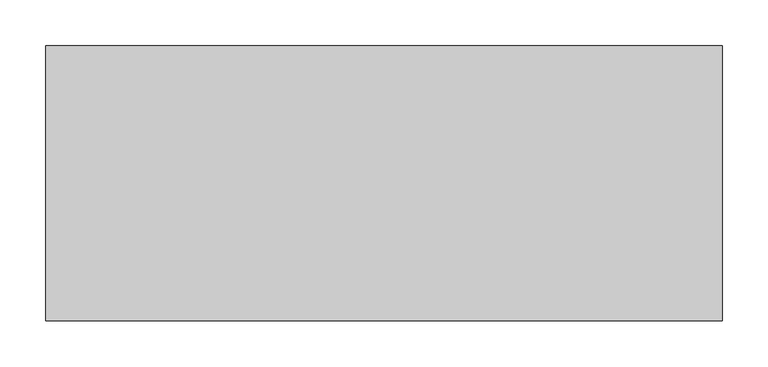
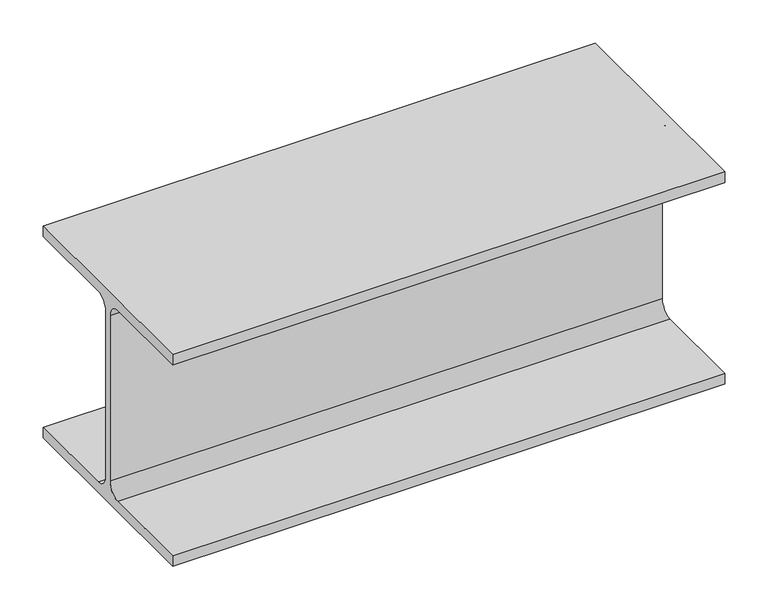
"""IFC4 building model written with IfcOpenShell, lengths in millimetres: beam geometry, 0912_Steel Framing_H-KSD3502 : H_SB_ASB_H-300x300x10x15."""

from ifc_helpers import new_model, si_unit, point, frame, frame_2d, origin, place, context, project, spatial, polyline, circle_curve, trimmed, segment, composite_curve, outline, extrude, source, transform, mapped, element, save


def beam_ffef67f5(model_context):
    return source(origin(), model_context, "Body", "SweptSolid", [
        extrude(outline(composite_curve([segment(polyline([(150.0, -135.0), (150.0, -150.0), (-150.0, -150.0), (-150.0, -135.0), (-23.0, -135.0)]), True, "CONTINUOUS"), segment(trimmed(circle_curve(frame_2d((-23.0, -117.0)), 18.0), [point((-23.0, -135.0))], [point((-5.0, -117.0))], True, "CARTESIAN"), True, "CONTINUOUS"), segment(polyline([(-5.0, -117.0), (-5.0, 117.0)]), True, "CONTINUOUS"), segment(trimmed(circle_curve(frame_2d((-23.0, 117.0)), 18.0), [point((-5.0, 117.0))], [point((-23.0, 135.0))], True, "CARTESIAN"), True, "CONTINUOUS"), segment(polyline([(-23.0, 135.0), (-150.0, 135.0), (-150.0, 150.0), (150.0, 150.0), (150.0, 135.0), (23.0, 135.0)]), True, "CONTINUOUS"), segment(trimmed(circle_curve(frame_2d((23.0, 117.0)), 18.0), [point((23.0, 135.0))], [point((5.0, 117.0))], True, "CARTESIAN"), True, "CONTINUOUS"), segment(polyline([(5.0, 117.0), (5.0, -117.0)]), True, "CONTINUOUS"), segment(trimmed(circle_curve(frame_2d((23.0, -117.0)), 18.0), [point((5.0, -117.0))], [point((23.0, -135.0))], True, "CARTESIAN"), True, "CONTINUOUS"), segment(polyline([(23.0, -135.0), (150.0, -135.0)]), True, "CONTINUOUS")], self_intersect=False)), frame((-502.4937811, 0.0, 0.0), z_axis=(1.0, 0.0, 0.0), x_axis=(0.0, 1.0, 0.0)), (0.0, 0.0, 1.0), 738.1005223),
    ])


if __name__ == "__main__":
    model = new_model("IFC4")
    model_context = context("Model", 3, world=origin())
    ifc_project = project(units=[si_unit("LENGTHUNIT", "METRE", prefix="MILLI")], contexts=[model_context])
    site = spatial("IfcSite", under=ifc_project)
    building = spatial("IfcBuilding", under=site)
    placement = place(None, origin())
    beam_shape = beam_ffef67f5(model_context)
    element("IfcBeam", 1, ObjectType="0912_Steel Framing_H-KSD3502 : H_SB_ASB_H-300x300x10x15", at=placement, inside=building, context=model_context, shape_type="MappedRepresentation", body=[
        mapped(beam_shape, transform((0.0, 0.0, 0.0), x_axis=(1.0, 0.0, 0.0), y_axis=(0.0, 1.0, 0.0), z_axis=(0.0, 0.0, 1.0))),
    ])
    save(model, "model.ifc")

# Revit data of these elements
# Type "0912_Steel Framing_H-KSD3502 : H_SB_ASB_H-300x300x10x15"
#   H_WM Code_1 = "S01AA001-00001 | Main Steel Structure Fabrication Work | Shelter/Building | Heavy Steel - Standard (Weight≥90KG/M) | Material: (   )"
#   H_WM Code_2 = "S03AA027-00001 | Main Steel Structure Erection Work | Shelter/Building | Heavy Steel (Weight≥90KG/M) | Material: (   )"
#   H_WM Code_3 = "S01AA010-00001 | Main Steel Structure Fabrication Work | Shelter/Building | Steel Painting/Coating | for Non-Fireproofed Steel Surface, Surface Preparation, Primer, Second & Final Coat | Material: (   )"
#   H_Q'ty Cal Type Tag = "SB-Q2"
#   Width = 30.0 cm
#   Web Thickness = 1.0 cm
#   Web Fillet = 1.8 cm
#   Warping Constant = 1370000.0 cm⁶
#   W = 0
#   Torsional Moment of Inertia = 77.00 cm⁴
#   Section Area = 119.8 cm²
#   Plastic Modulus weak axis = 684.0 cm³
#   Plastic Modulus strong axis = 1500.0 cm³
#   Perimeter = 1.75 m²/m
#   Nominal Weight = 94.00 kgf/m
#   Moment of Inertia weak axis = 6750.00 cm⁴
#   Moment of Inertia strong axis = 20400.00 cm⁴
#   Height = 30.0 cm
#   Flange Thickness = 1.5 cm
#   Elastic Modulus weak axis = 450.0 cm³
#   Elastic Modulus strong axis = 1360.0 cm³
#   Centroid Vertical = 15.0 cm
#   Centroid Horizontal = 15.0 cm
#   Ix = 204000000
#   Length [instance default] = 1.5240 m
#   Zx = 1500000
#   b = 0.3000 m
#   h = 0.3000 m
#   r = 0.0180 m
#   s = 0.0100 m
#   t = 0.0150 m
#   A = 0.01198 m²
#   Structural Material [instance default] = Steel, 45-345
#   Assembly Code = ""
# Element 1 (IfcBeam, "0912_Steel Framing_H-KSD3502 : H_SB_ASB_H-300x300x10x15")
#   Structural Material = none
# Materials
#   "Steel, 45-345": class "Metal", colour RGB 189 187 185, transparency 0, Description = "Steel 345 MPa", Cost = 0
